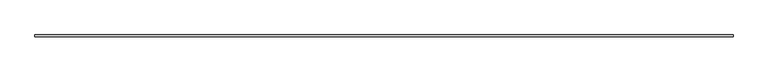
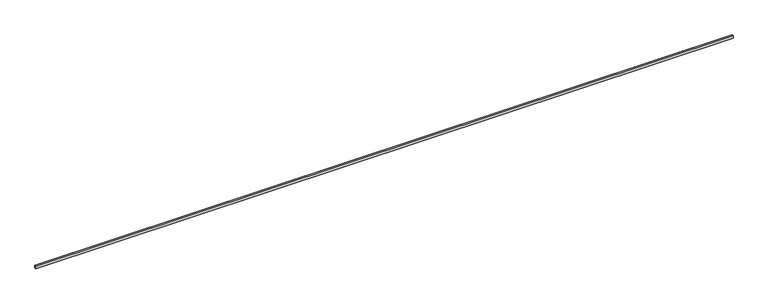
"""IFC4 building model written with IfcOpenShell, lengths in millimetres: proxy geometry, Generic Models 3:Generic Models 2:312240:Generic Models 2:312240 : Generic Models 3:Generic Models 2:312240:12 : Generic Models 3:Generic Models 2:312240:Generic Models 2:312240 : Generic Models 3:Generic Models 2:312240:300533."""

from ifc_helpers import new_model, si_unit, frame, origin, place, context, project, spatial, polyline, outline, extrude, source, transform, mapped, element, save


def generic_models_233170d9(model_context):
    return source(origin(), model_context, "Body", "SweptSolid", [
        extrude(outline(polyline([(-579008.3631464, 1180.9715625), (-579010.5010917, 1181.5444232), (-579011.9127678, 1181.2955066), (-579013.3913841, 1179.8168903), (-579013.3913841, 1188.6216337), (-579007.0413841, 1188.6216337), (-579007.0413841, 1180.0460545), (-579008.3631464, 1180.9715625)])), frame((590317.0242239, 0.0, 0.0), z_axis=(1.0, 0.0, 0.0), x_axis=(0.0, 1.0, 0.0)), (0.0, 0.0, 1.0), 2438.4),
    ])


if __name__ == "__main__":
    model = new_model("IFC4")
    model_context = context("Model", 3, world=origin())
    ifc_project = project(units=[si_unit("LENGTHUNIT", "METRE", prefix="MILLI")], contexts=[model_context])
    site = spatial("IfcSite", under=ifc_project)
    building = spatial("IfcBuilding", under=site)
    placement = place(None, origin())
    generic_models_shape = generic_models_233170d9(model_context)
    element("IfcBuildingElementProxy", 1, Name="Generic Models 3:Generic Models 2:312240:Generic Models 2:312240 : Generic Models 3:Generic Models 2:312240:12 : Generic Models 3:Generic Models 2:312240:Generic Models 2:312240 : Generic Models 3:Generic Models 2:312240:300533", ObjectType="Generic Models 3:Generic Models 2:312240:Generic Models 2:312240 : Generic Models 3:Generic Models 2:312240:12 : Generic Models 3:Generic Models 2:312240:Generic Models 2:312240 : Generic Models 3:Generic Models 2:312240:300533", at=placement, inside=building, context=model_context, shape_type="MappedRepresentation", body=[
        mapped(generic_models_shape, transform((0.0, 0.0, 0.0), x_axis=(1.0, 0.0, 0.0), y_axis=(0.0, 1.0, 0.0), z_axis=(0.0, 0.0, 1.0))),
    ])
    save(model, "model.ifc")

# Revit data of these elements
# Type "Generic Models 3:Generic Models 2:312240:Generic Models 2:312240 : Generic Models 3:Generic Models 2:312240:12 : Generic Models 3:Generic Models 2:312240:Generic Models 2:312240 : Generic Models 3:Generic Models 2:312240:300533"
#   NameOverride = "Generic Models 3:Generic Models 2:312240:Generic Models 2:312240 : Generic Models 3:Generic Models 2:312240:300533"
#   ObjectTypeOverride = "Generic Models 2:312240 : Generic Models 3:Generic Models 2:312240"
#   Reference = "Generic Models 2"
#   Tag = "300533"
# Element 1 (IfcBuildingElementProxy, "Generic Models 3:Generic Models 2:312240:Generic Models 2:312240 : Generic Models 3:Generic Models 2:312240:12 : Generic Models 3:Generic Models 2:312240:Generic Models 2:312240 : Generic Models 3:Generic Models 2:312240:300533")
#   Materials on its faces: "SILICONE SEALANT"
# Materials
#   "SILICONE SEALANT": class "Generic", colour RGB 221 221 221, transparency 0, Cost = 0
